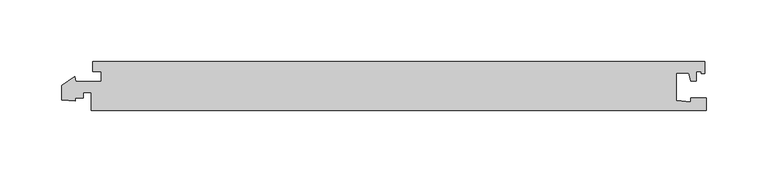
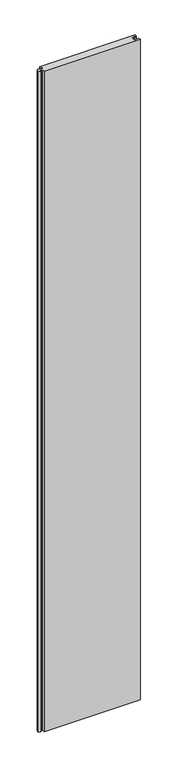
"""IFC4 building model written with IfcOpenShell, lengths in millimetres: proxy geometry, Generic Models 5:Generic Models 5:321804:Generic Models 5:321804 : Generic Models 5:Generic Models 5:321804:2 : Generic Models 5:Generic Models 5:321804:Generic Models 5:321804 : Generic Models 5:Generic Models 5:321804:300761."""

from ifc_helpers import new_model, si_unit, frame, origin, place, context, project, spatial, polyline, outline, extrude, source, transform, mapped, element, save


def generic_models_2f3a26a6(model_context):
    return source(origin(), model_context, "Body", "SweptSolid", [
        extrude(outline(polyline([(592220.2261126, -579052.1037319), (592209.8677824, -579052.1037319), (592209.8677824, -579074.5995222), (592221.8677824, -579075.6493861), (592221.8677824, -579072.4037319), (592234.6177824, -579072.4037319), (592234.6177824, -579082.6037319), (591734.6177824, -579082.6037319), (591734.6177824, -579068.1037319), (591727.9927824, -579068.1037319), (591727.9927824, -579072.4037319), (591721.3677824, -579072.4037319), (591721.3677824, -579075.1037319), (591710.3677824, -579074.1413566), (591710.3677824, -579062.2832156), (591721.0492843, -579055.1758504), (591722.101757, -579059.1037319), (591742.8177824, -579059.1037319), (591742.8177824, -579051.1037319), (591735.8677824, -579051.1037319), (591735.8677824, -579042.6037319), (592233.3677824, -579042.6037319), (592233.3677824, -579052.6037319), (592230.3677824, -579052.6037319), (592230.3677824, -579051.1037319), (592226.4177824, -579051.1037319), (592226.4177824, -579058.6037319), (592221.9677824, -579058.6037319), (592220.2261126, -579052.1037319)])), frame((0.0, 0.0, 30.0324973), z_axis=(0.0, 0.0, 1.0), x_axis=(1.0, 0.0, 0.0)), (0.0, 0.0, 1.0), 3634.8310765),
    ])


if __name__ == "__main__":
    model = new_model("IFC4")
    model_context = context("Model", 3, world=origin())
    ifc_project = project(units=[si_unit("LENGTHUNIT", "METRE", prefix="MILLI")], contexts=[model_context])
    site = spatial("IfcSite", under=ifc_project)
    building = spatial("IfcBuilding", under=site)
    placement = place(None, origin())
    generic_models_shape = generic_models_2f3a26a6(model_context)
    element("IfcBuildingElementProxy", 1, Name="Generic Models 5:Generic Models 5:321804:Generic Models 5:321804 : Generic Models 5:Generic Models 5:321804:2 : Generic Models 5:Generic Models 5:321804:Generic Models 5:321804 : Generic Models 5:Generic Models 5:321804:300761", ObjectType="Generic Models 5:Generic Models 5:321804:Generic Models 5:321804 : Generic Models 5:Generic Models 5:321804:2 : Generic Models 5:Generic Models 5:321804:Generic Models 5:321804 : Generic Models 5:Generic Models 5:321804:300761", at=placement, inside=building, context=model_context, shape_type="MappedRepresentation", body=[
        mapped(generic_models_shape, transform((0.0, 0.0, 0.0), x_axis=(1.0, 0.0, 0.0), y_axis=(0.0, 1.0, 0.0), z_axis=(0.0, 0.0, 1.0))),
    ])
    save(model, "model.ifc")

# Revit data of these elements
# Type "Generic Models 5:Generic Models 5:321804:Generic Models 5:321804 : Generic Models 5:Generic Models 5:321804:2 : Generic Models 5:Generic Models 5:321804:Generic Models 5:321804 : Generic Models 5:Generic Models 5:321804:300761"
#   NameOverride = "Generic Models 5:Generic Models 5:321804:Generic Models 5:321804 : Generic Models 5:Generic Models 5:321804:300761"
#   ObjectTypeOverride = "Generic Models 5:321804 : Generic Models 5:Generic Models 5:321804"
#   Reference = "Generic Models 5"
#   Tag = "300761"
# Element 1 (IfcBuildingElementProxy, "Generic Models 5:Generic Models 5:321804:Generic Models 5:321804 : Generic Models 5:Generic Models 5:321804:2 : Generic Models 5:Generic Models 5:321804:Generic Models 5:321804 : Generic Models 5:Generic Models 5:321804:300761")
#   Materials on its faces: "POLYCARBONATE PANEL - ARCOPLUS 547"
# Materials
#   "POLYCARBONATE PANEL - ARCOPLUS 547": class "Unassigned", colour RGB 202 225 249, transparency 0.45, Cost = 0
